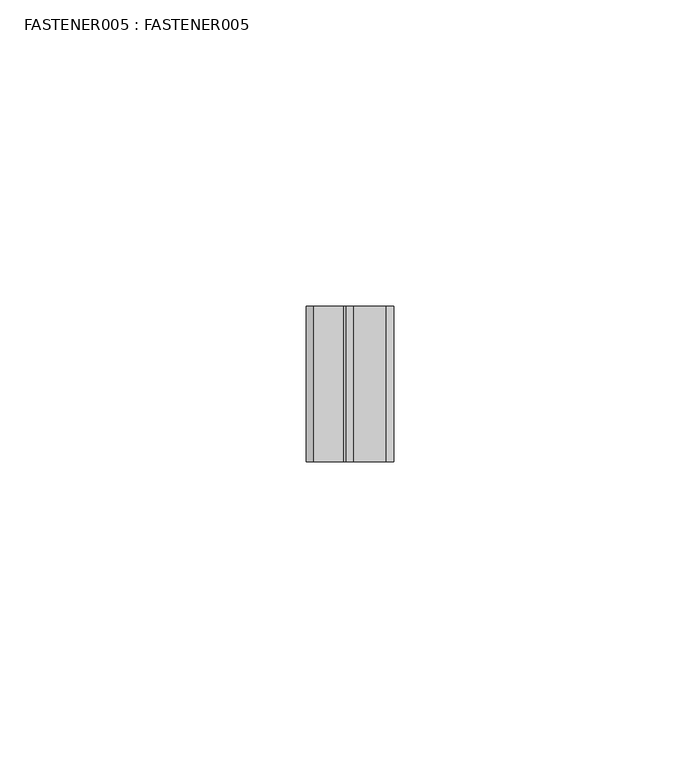
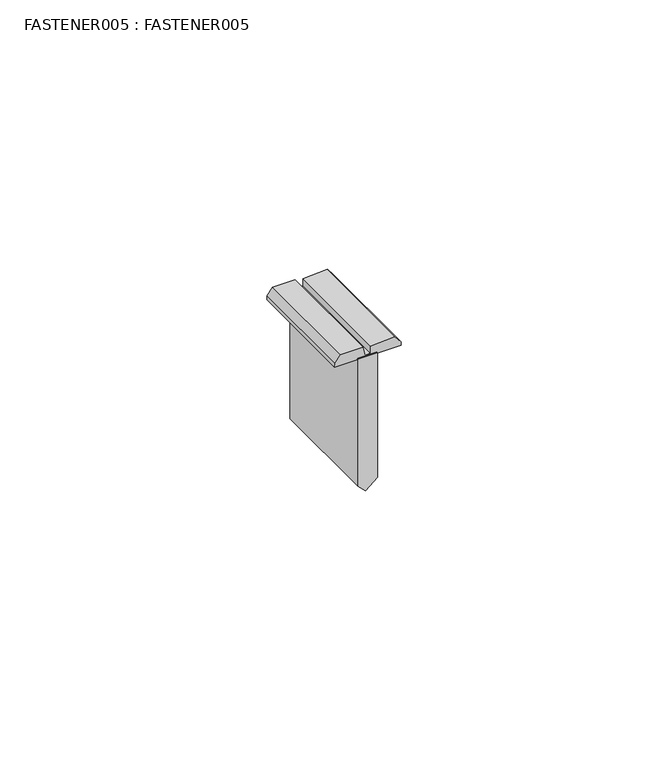
"""IFC4 building model written with IfcOpenShell, lengths in millimetres: proxy geometry, FASTENER005 : FASTENER005."""

import ifcopenshell
import ifcopenshell.guid

model = None  # the IFC model being written
_history = None  # IfcOwnerHistory: only IFC2X3 demands one
_inside = {}  # id of a spatial element -> (the spatial element, [elements in it])
_under = {}  # id of a project, library or spatial element -> (it, [spatial elements below it])
_declared = {}  # id of a project -> (the project, [libraries it declares])
_typed = {}  # id of a type object -> (the type object, [elements of that type])
_made_of = {}  # id of a material, layer set ... -> (it, [elements and type objects made of it])


def new_model(schema):
    """Start an empty IFC model of exactly this schema.

    Asked for "IFC4X3", IfcOpenShell would pick the latest addendum, in which some entities
    have other attributes; the version numbers below select the first issue.
    IFC2X3 requires an IfcOwnerHistory on every rooted entity: one is made here for all.
    """
    global model, _history
    if schema == "IFC4X3":
        model = ifcopenshell.file(schema_version=(4, 3, 0, 0))
    else:
        model = ifcopenshell.file(schema=schema)
    _inside.clear()
    _under.clear()
    _declared.clear()
    _typed.clear()
    _made_of.clear()
    _history = None
    if model.schema == "IFC2X3":
        org = make("IfcOrganization", Name="unknown")
        user = make(
            "IfcPersonAndOrganization",
            ThePerson=make("IfcPerson", FamilyName="unknown"),
            TheOrganization=org,
        )
        app = make(
            "IfcApplication",
            ApplicationDeveloper=org,
            Version="unknown",
            ApplicationFullName="unknown",
            ApplicationIdentifier="unknown",
        )
        _history = make(
            "IfcOwnerHistory",
            OwningUser=user,
            OwningApplication=app,
            ChangeAction="ADDED",
            CreationDate=0,
        )
    return model


def make(cls, **values):
    """One entity of the class cls with the attributes given. An attribute that is None is left unset."""
    return model.create_entity(
        cls, **{name: value for name, value in values.items() if value is not None}
    )


def rooted(cls, **values):
    """An entity with a GlobalId (a new one), such as an element, a storey or a relation."""
    return make(cls, GlobalId=ifcopenshell.guid.new(), OwnerHistory=_history, **values)


def si_unit(unit_type, name, prefix=None):
    """IfcSIUnit, for example si_unit("LENGTHUNIT", "METRE", prefix="MILLI")."""
    return make("IfcSIUnit", UnitType=unit_type, Prefix=prefix, Name=name)


def assignment(units):
    """IfcUnitAssignment: the units of a project."""
    return None if units is None else make("IfcUnitAssignment", Units=units)


def point(xyz):
    """IfcCartesianPoint."""
    return None if xyz is None else make("IfcCartesianPoint", Coordinates=xyz)


def direction(xyz):
    """IfcDirection."""
    return None if xyz is None else make("IfcDirection", DirectionRatios=xyz)


def frame(location, z_axis=None, x_axis=None):
    """IfcAxis2Placement3D, a coordinate frame: its origin and axes. An axis left out is left unset."""
    return make(
        "IfcAxis2Placement3D",
        Location=point(location),
        Axis=direction(z_axis),
        RefDirection=direction(x_axis),
    )


def origin():
    """The frame at (0, 0, 0) with its axes left unset."""
    return frame((0.0, 0.0, 0.0))


def place(relative_to, where):
    """IfcLocalPlacement: puts the frame where relative to a parent placement (None: the world)."""
    return make(
        "IfcLocalPlacement", PlacementRelTo=relative_to, RelativePlacement=where
    )


def context(
    kind, dimensions, precision=None, world=None, true_north=None, identifier=None
):
    """IfcGeometricRepresentationContext, for example the 3D "Model" context."""
    return make(
        "IfcGeometricRepresentationContext",
        ContextIdentifier=identifier,
        ContextType=kind,
        CoordinateSpaceDimension=dimensions,
        Precision=precision,
        WorldCoordinateSystem=world,
        TrueNorth=true_north,
    )


def project(units=None, contexts=None):
    """IfcProject with its units and contexts."""
    return rooted(
        "IfcProject",
        Name="project",
        RepresentationContexts=contexts,
        UnitsInContext=assignment(units),
    )


def spatial(cls, under=None, at=None, **own):
    """A site, building, storey or space (cls), placed at a placement, below another one or the project."""
    s = rooted(cls, ObjectPlacement=at, **own)
    if under is not None:
        _under.setdefault(under.id(), (under, []))[1].append(s)
    return s


def polyline(points):
    """IfcPolyline through the points."""
    return make("IfcPolyline", Points=[point(p) for p in points])


def outline(outer, holes=None, kind="AREA"):
    """IfcArbitraryClosedProfileDef: a profile drawn as a closed curve; with holes, ...WithVoids."""
    if holes is None:
        return make("IfcArbitraryClosedProfileDef", ProfileType=kind, OuterCurve=outer)
    return make(
        "IfcArbitraryProfileDefWithVoids",
        ProfileType=kind,
        OuterCurve=outer,
        InnerCurves=holes,
    )


def extrude(swept, where, along, depth):
    """IfcExtrudedAreaSolid: the profile swept, set in the frame where, extruded along a direction by depth."""
    return make(
        "IfcExtrudedAreaSolid",
        SweptArea=swept,
        Position=where,
        ExtrudedDirection=direction(along),
        Depth=depth,
    )


def shape(context_of_items, identifier, shape_type, items):
    """IfcShapeRepresentation: the items that make up one representation, for example the "Body"."""
    return make(
        "IfcShapeRepresentation",
        ContextOfItems=context_of_items,
        RepresentationIdentifier=identifier,
        RepresentationType=shape_type,
        Items=items,
    )


def source(mapping_origin, context_of_items, identifier, shape_type, items):
    """IfcRepresentationMap: a shape defined once, which mapped items show again and again."""
    return make(
        "IfcRepresentationMap",
        MappingOrigin=mapping_origin,
        MappedRepresentation=shape(context_of_items, identifier, shape_type, items),
    )


def transform(
    local_origin,
    x_axis=None,
    y_axis=None,
    z_axis=None,
    scale=None,
    scale2=None,
    scale3=None,
    uniform=True,
):
    """IfcCartesianTransformationOperator3D, or its non-uniform kind. x_axis, y_axis, z_axis: its Axis1, 2, 3."""
    if uniform:
        return make(
            "IfcCartesianTransformationOperator3D",
            Axis1=direction(x_axis),
            Axis2=direction(y_axis),
            LocalOrigin=point(local_origin),
            Scale=scale,
            Axis3=direction(z_axis),
        )
    return make(
        "IfcCartesianTransformationOperator3DnonUniform",
        Axis1=direction(x_axis),
        Axis2=direction(y_axis),
        LocalOrigin=point(local_origin),
        Scale=scale,
        Axis3=direction(z_axis),
        Scale2=scale2,
        Scale3=scale3,
    )


def mapped(mapping_source, mapping_target):
    """IfcMappedItem: shows the shape of a source again, moved by a transform."""
    return make(
        "IfcMappedItem", MappingSource=mapping_source, MappingTarget=mapping_target
    )


def made_of(thing, what):
    """Note that an element or type object is made of a material, layer set ...; save() writes the relation."""
    if what is not None:
        _made_of.setdefault(what.id(), (what, []))[1].append(thing)
    return thing


def element(
    cls,
    number,
    at=None,
    inside=None,
    cuts=None,
    type_object=None,
    material=None,
    context=None,
    identifier="Body",
    shape_type=None,
    held_by="IfcProductDefinitionShape",
    body=None,
    shapes=None,
    **own,
):
    """One element of the class cls, such as IfcWall. Its Tag is "e" and its number.

    at: its placement. inside: the storey or other place that contains it. cuts: it is an
    opening in that element (IfcRelVoidsElement). A single representation is given by context,
    identifier, shape_type and body (its items); several are given by shapes. held_by: the class
    of the entity that holds the representations. save() writes the other relations.
    """
    e = rooted(cls, Tag="e%d" % number, ObjectPlacement=at, **own)
    if body is not None:
        shapes = [shape(context, identifier, shape_type, body)]
    if shapes is not None:
        e.Representation = make(held_by, Representations=shapes)
    if inside is not None:
        _inside.setdefault(inside.id(), (inside, []))[1].append(e)
    if cuts is not None:
        rooted(
            "IfcRelVoidsElement", RelatingBuildingElement=cuts, RelatedOpeningElement=e
        )
    if type_object is not None:
        _typed.setdefault(type_object.id(), (type_object, []))[1].append(e)
    return made_of(e, material)


def aggregate(whole, parts):
    """IfcRelAggregates: a whole, such as a stair, and the parts it consists of."""
    return rooted("IfcRelAggregates", RelatingObject=whole, RelatedObjects=parts)


def save(model, path):
    """Write the relations noted so far, then the file.

    IfcRelAggregates (storeys below a building ...), IfcRelContainedInSpatialStructure (elements
    in a storey), IfcRelDefinesByType, IfcRelAssociatesMaterial and IfcRelDeclares: one each for
    every whole, place, type object, material and project.
    """
    for whole, parts in _under.values():
        aggregate(whole, parts)
    for where, things in _inside.values():
        rooted(
            "IfcRelContainedInSpatialStructure",
            RelatedElements=things,
            RelatingStructure=where,
        )
    for kind, things in _typed.values():
        rooted("IfcRelDefinesByType", RelatedObjects=things, RelatingType=kind)
    for what, things in _made_of.values():
        rooted("IfcRelAssociatesMaterial", RelatedObjects=things, RelatingMaterial=what)
    for by, libraries in _declared.values():
        rooted("IfcRelDeclares", RelatingContext=by, RelatedDefinitions=libraries)
    model.write(path)


def fastener005_fastener005_4a0cef2c(model_context):
    return source(origin(), model_context, "Body", "SweptSolid", [
        extrude(outline(polyline([(42579.6987049, 5977.3107075), (42550.7399648, 5977.3107075), (42549.1244121, 5978.9677221), (42551.3049701, 5981.517626), (42579.6987049, 5981.517626), (42579.6987049, 5977.3107075)])), frame((0.0, -1078.2906574, 0.0), z_axis=(0.0, 1.0, 0.0), x_axis=(0.0, 0.0, 1.0)), (0.0, 0.0, 1.0), 25.4),
        extrude(outline(polyline([(42579.6987049, 5986.5634932), (42580.508527, 5986.5634932), (42582.1023984, 5985.3247911), (42581.7061629, 5980.0391089), (42580.1167322, 5980.0391089), (42580.1167322, 5978.792004), (42582.1288635, 5978.3957685), (42582.1288635, 5973.5166866), (42580.5349921, 5972.2779845), (42579.6987049, 5972.2671879), (42579.6987049, 5986.5634932)])), frame((0.0, -1078.2906574, 0.0), z_axis=(0.0, 1.0, 0.0), x_axis=(0.0, 0.0, 1.0)), (0.0, 0.0, 1.0), 25.4),
    ])


if __name__ == "__main__":
    model = new_model("IFC4")
    model_context = context("Model", 3, world=origin())
    ifc_project = project(units=[si_unit("LENGTHUNIT", "METRE", prefix="MILLI")], contexts=[model_context])
    site = spatial("IfcSite", under=ifc_project)
    building = spatial("IfcBuilding", under=site)
    placement = place(None, origin())
    fastener005_fastener005_shape = fastener005_fastener005_4a0cef2c(model_context)
    element("IfcBuildingElementProxy", 1, Name="FASTENER005 : FASTENER005", ObjectType="FASTENER005 : FASTENER005", at=placement, inside=building, context=model_context, shape_type="MappedRepresentation", body=[
        mapped(fastener005_fastener005_shape, transform((0.0, 0.0, 0.0), x_axis=(1.0, 0.0, 0.0), y_axis=(0.0, 1.0, 0.0), z_axis=(0.0, 0.0, 1.0))),
    ])
    save(model, "model.ifc")

# Revit data of these elements
# Type "FASTENER005 : FASTENER005"
#   NameOverride = "FASTENER005"
# Element 1 (IfcBuildingElementProxy, "FASTENER005 : FASTENER005")
#   Materials on its faces: "ENGINEERED PANCAKE HEAD FASTENER @ 12\" O.C."
# Materials
#   "ENGINEERED PANCAKE HEAD FASTENER @ 12\" O.C.": class "Unassigned", colour RGB 255 255 255, transparency 0, Cost = 0
